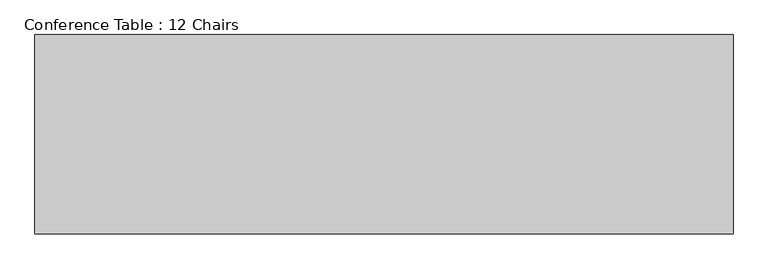
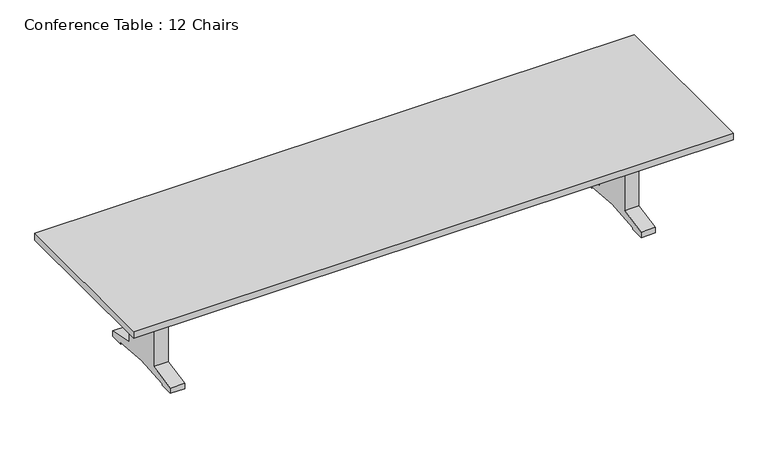
"""IFC4 building model written with IfcOpenShell, lengths in millimetres: furniture geometry, Conference Table : 12 Chairs."""

from ifc_helpers import new_model, si_unit, frame, origin, place, context, project, spatial, polyline, outline, extrude, source, transform, mapped, element, save


def conference_table_12_chairs_3d940985(model_context):
    return source(origin(), model_context, "Body", "SweptSolid", [
        extrude(outline(polyline([(-254.0, 0.0), (-355.6, 0.0), (-355.6, 40.4390459), (-152.4, 79.9371247), (-152.4, 555.8555363), (-457.2, 609.6), (-457.2, 711.2), (457.2, 711.2), (457.2, 609.6), (152.4, 555.8555363), (152.4, 79.9371247), (355.6, 40.4390459), (355.6, 0.0), (254.0, 0.0), (254.0, 12.7), (0.0, 34.9221205), (-254.0, 12.7), (-254.0, 0.0)])), frame((1625.6, 0.0, 0.0), z_axis=(1.0, 0.0, 0.0), x_axis=(0.0, 1.0, 0.0)), (0.0, 0.0, 1.0), 101.6),
        extrude(outline(polyline([(-254.0, 0.0), (-355.6, 0.0), (-355.6, 40.4390459), (-152.4, 79.9371247), (-152.4, 555.8555363), (-457.2, 609.6), (-457.2, 711.2), (457.2, 711.2), (457.2, 609.6), (152.4, 555.8555363), (152.4, 79.9371247), (355.6, 40.4390459), (355.6, 0.0), (254.0, 0.0), (254.0, 12.7), (0.0, 34.9221205), (-254.0, 12.7), (-254.0, 0.0)])), frame((-1727.2, 0.0, 0.0), z_axis=(1.0, 0.0, 0.0), x_axis=(0.0, 1.0, 0.0)), (0.0, 0.0, 1.0), 101.6),
        extrude(outline(polyline([(2133.6, -609.6), (-2133.6, -609.6), (-2133.6, 609.6), (2133.6, 609.6), (2133.6, -609.6)])), frame((0.0, 0.0, 711.2), z_axis=(0.0, 0.0, 1.0), x_axis=(1.0, 0.0, 0.0)), (0.0, 0.0, 1.0), 50.8),
        extrude(outline(polyline([(1625.6, 457.2), (1625.6, 419.1), (-1625.6, 419.1), (-1625.6, 457.2), (1625.6, 457.2)])), frame((0.0, 0.0, 609.6), z_axis=(0.0, 0.0, 1.0), x_axis=(1.0, 0.0, 0.0)), (0.0, 0.0, 1.0), 101.6),
        extrude(outline(polyline([(1625.6, -457.2), (-1625.6, -457.2), (-1625.6, -419.1), (1625.6, -419.1), (1625.6, -457.2)])), frame((0.0, 0.0, 609.6), z_axis=(0.0, 0.0, 1.0), x_axis=(1.0, 0.0, 0.0)), (0.0, 0.0, 1.0), 101.6),
    ])


if __name__ == "__main__":
    model = new_model("IFC4")
    model_context = context("Model", 3, world=origin())
    ifc_project = project(units=[si_unit("LENGTHUNIT", "METRE", prefix="MILLI")], contexts=[model_context])
    site = spatial("IfcSite", under=ifc_project)
    building = spatial("IfcBuilding", under=site)
    placement = place(None, origin())
    conference_table_12_chairs_shape = conference_table_12_chairs_3d940985(model_context)
    element("IfcFurniture", 1, ObjectType="Conference Table : 12 Chairs", at=placement, inside=building, context=model_context, shape_type="MappedRepresentation", body=[
        mapped(conference_table_12_chairs_shape, transform((0.0, 0.0, 0.0), x_axis=(1.0, 0.0, 0.0), y_axis=(0.0, 1.0, 0.0), z_axis=(0.0, 0.0, 1.0))),
    ])
    save(model, "model.ifc")

# Revit data of these elements
# Type "Conference Table : 12 Chairs"
#   Model = "TBL-12CH"
#   Manufacturer = "Acme Furniture"
#   Type Mark = "TB-2"
#   Cost = 9250
#   Width = 4' - 0"
#   Length = 14' - 0"
#   Height = 2' - 6"
#   Number of Chairs = 12
#   Number Of Chairs One Side = 5
#   Top = Mahogany
#   Legs and Supports = Mahogany
#   Default Elevation = 0
# Element 1 (IfcFurniture, "Conference Table : 12 Chairs")
#   Materials on its faces: "Mahogany"
# Materials
#   "Mahogany": class "Wood", colour RGB 102 51 32, transparency 0, Description = "Swietenia Macrophylla", Cost = 0
